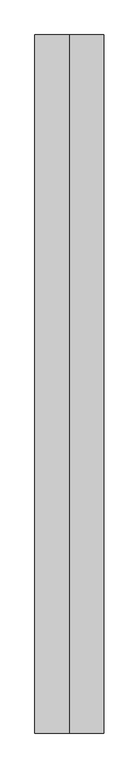
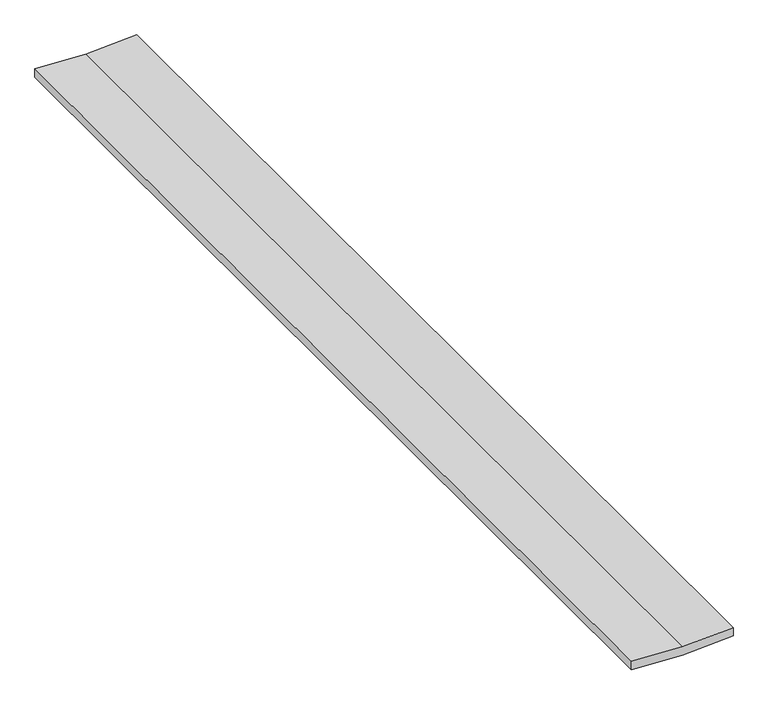
"""IFC4 building model written with IfcOpenShell, lengths in millimetres: proxy geometry, COVER BOARD3:COVER BOARD001:300174 : COVER BOARD3:COVER BOARD001:300174."""

from ifc_helpers import new_model, si_unit, frame, origin, place, context, project, spatial, polyline, outline, extrude, source, transform, mapped, element, save


def generic_models_5e33c8b1(model_context):
    return source(origin(), model_context, "Body", "SweptSolid", [
        extrude(outline(polyline([(40233.346, 175.9552255), (40228.3444286, 77.2027316), (40233.346, -20.8947745), (40216.0142809, -20.8947745), (40211.0127094, 77.2027316), (40216.0142809, 175.9552255), (40233.346, 175.9552255)])), frame((0.0, -774.3081162, 0.0), z_axis=(0.0, 1.0, 0.0), x_axis=(0.0, 0.0, 1.0)), (0.0, 0.0, 1.0), 2000.0),
    ])


if __name__ == "__main__":
    model = new_model("IFC4")
    model_context = context("Model", 3, world=origin())
    ifc_project = project(units=[si_unit("LENGTHUNIT", "METRE", prefix="MILLI")], contexts=[model_context])
    site = spatial("IfcSite", under=ifc_project)
    building = spatial("IfcBuilding", under=site)
    placement = place(None, origin())
    generic_models_shape = generic_models_5e33c8b1(model_context)
    element("IfcBuildingElementProxy", 1, Name="COVER BOARD3:COVER BOARD001:300174 : COVER BOARD3:COVER BOARD001:300174", ObjectType="COVER BOARD3:COVER BOARD001:300174 : COVER BOARD3:COVER BOARD001:300174", at=placement, inside=building, context=model_context, shape_type="MappedRepresentation", body=[
        mapped(generic_models_shape, transform((0.0, 0.0, 0.0), x_axis=(1.0, 0.0, 0.0), y_axis=(0.0, 1.0, 0.0), z_axis=(0.0, 0.0, 1.0))),
    ])
    save(model, "model.ifc")

# Revit data of these elements
# Type "COVER BOARD3:COVER BOARD001:300174 : COVER BOARD3:COVER BOARD001:300174"
#   NameOverride = "COVER BOARD3:COVER BOARD001:300174"
#   ObjectTypeOverride = "COVER BOARD3:COVER BOARD001"
#   Reference = "COVER BOARD001"
#   Category = "Generic Models"
#   Tag = "300174"
# Element 1 (IfcBuildingElementProxy, "COVER BOARD3:COVER BOARD001:300174 : COVER BOARD3:COVER BOARD001:300174")
#   Materials on its faces: "CDX PLYWOOD - SEE STRUCTURAL DWGS"
# Materials
#   "CDX PLYWOOD - SEE STRUCTURAL DWGS": class "Unassigned", colour RGB 202 163 108, transparency 0, Cost = 0
